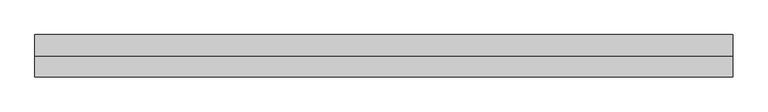
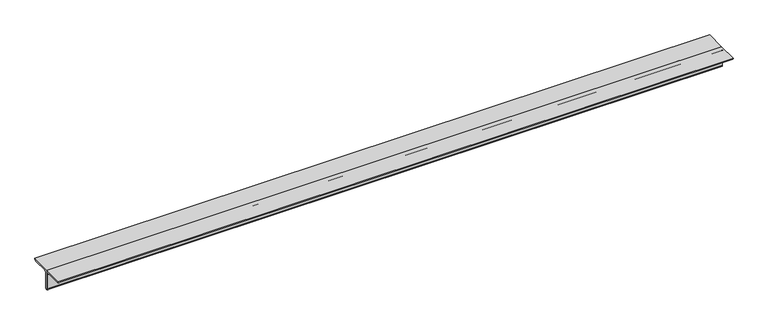
"""IFC4 building model written with IfcOpenShell, lengths in millimetres: member geometry, 0123_Steel Framing_2Ls-KSD3502 : H_SB_AR_S03_2Ls-130x130x12_HBR4."""

from ifc_helpers import new_model, si_unit, point, frame, frame_2d, origin, place, context, project, spatial, polyline, circle_curve, trimmed, segment, composite_curve, outline, extrude, source, transform, mapped, element, save


def member_26d310ba(model_context):
    return source(origin(), model_context, "Body", "SweptSolid", [
        extrude(outline(composite_curve([segment(polyline([(0.0, 36.4), (130.0, 36.4)]), True, "CONTINUOUS"), segment(trimmed(circle_curve(frame_2d((118.0, 36.4)), 12.0), [point((130.0, 36.4))], [point((118.0, 24.4))], False, "CARTESIAN"), True, "CONTINUOUS"), segment(polyline([(118.0, 24.4), (24.0, 24.4)]), True, "CONTINUOUS"), segment(trimmed(circle_curve(frame_2d((24.0, 12.4)), 12.0), [point((24.0, 24.4))], [point((12.0, 12.4))], True, "CARTESIAN"), True, "CONTINUOUS"), segment(polyline([(12.0, 12.4), (12.0, -81.6)]), True, "CONTINUOUS"), segment(trimmed(circle_curve(frame_2d((0.0, -81.6)), 12.0), [point((12.0, -81.6))], [point((0.0, -93.6))], False, "CARTESIAN"), True, "CONTINUOUS"), segment(polyline([(0.0, -93.6), (0.0, 36.4)]), True, "CONTINUOUS")], self_intersect=False)), frame((-2215.9, 0.0, 0.0), z_axis=(1.0, 0.0, 0.0), x_axis=(0.0, 1.0, 0.0)), (0.0, 0.0, 1.0), 4294.8666667),
        extrude(outline(composite_curve([segment(polyline([(0.0, 36.4), (0.0, -93.6)]), True, "CONTINUOUS"), segment(trimmed(circle_curve(frame_2d((0.0, -81.6)), 12.0), [point((0.0, -93.6))], [point((-12.0, -81.6))], False, "CARTESIAN"), True, "CONTINUOUS"), segment(polyline([(-12.0, -81.6), (-12.0, 12.4)]), True, "CONTINUOUS"), segment(trimmed(circle_curve(frame_2d((-24.0, 12.4)), 12.0), [point((-12.0, 12.4))], [point((-24.0, 24.4))], True, "CARTESIAN"), True, "CONTINUOUS"), segment(polyline([(-24.0, 24.4), (-118.0, 24.4)]), True, "CONTINUOUS"), segment(trimmed(circle_curve(frame_2d((-118.0, 36.4)), 12.0), [point((-118.0, 24.4))], [point((-130.0, 36.4))], False, "CARTESIAN"), True, "CONTINUOUS"), segment(polyline([(-130.0, 36.4), (0.0, 36.4)]), True, "CONTINUOUS")], self_intersect=False)), frame((-2215.9, 0.0, 0.0), z_axis=(1.0, 0.0, 0.0), x_axis=(0.0, 1.0, 0.0)), (0.0, 0.0, 1.0), 4294.8666667),
    ])


if __name__ == "__main__":
    model = new_model("IFC4")
    model_context = context("Model", 3, world=origin())
    ifc_project = project(units=[si_unit("LENGTHUNIT", "METRE", prefix="MILLI")], contexts=[model_context])
    site = spatial("IfcSite", under=ifc_project)
    building = spatial("IfcBuilding", under=site)
    placement = place(None, origin())
    member_shape = member_26d310ba(model_context)
    element("IfcMember", 1, ObjectType="0123_Steel Framing_2Ls-KSD3502 : H_SB_AR_S03_2Ls-130x130x12_HBR4", at=placement, inside=building, context=model_context, shape_type="MappedRepresentation", body=[
        mapped(member_shape, transform((0.0, 0.0, 0.0), x_axis=(1.0, 0.0, 0.0), y_axis=(0.0, 1.0, 0.0), z_axis=(0.0, 0.0, 1.0))),
    ])
    save(model, "model.ifc")

# Revit data of these elements
# Type "0123_Steel Framing_2Ls-KSD3502 : H_SB_AR_S03_2Ls-130x130x12_HBR4"
#   Assembly Code = "B10"
#   Legs = "SLBB"
#   W = 8.97
#   Perimeter = 1.04 m²/m
#   Nominal Weight = 46.80 kgf/m
#   Length [instance default] = 1000 mm
#   Space = 0 mm
#   b = 130 mm
#   d = 130 mm
#   t = 12 mm
#   y = 36.4 mm
#   A = 0.005952 m²
#   Structural Material [instance default] = Steel ASTM A36
# Element 1 (IfcMember, "0123_Steel Framing_2Ls-KSD3502 : H_SB_AR_S03_2Ls-130x130x12_HBR4")
#   Structural Material = Steel, 45-345
#   Materials on its faces: "Steel, 45-345"
# Materials
#   "Steel ASTM A36": class "Metal", colour RGB 199 199 199, transparency 0, Description = "Structural steel, ASTM A36 Grade B, mill finish", Cost = 0
#   "Steel, 45-345": class "Metal", colour RGB 189 187 185, transparency 0, Description = "Steel 345 MPa", Cost = 0
